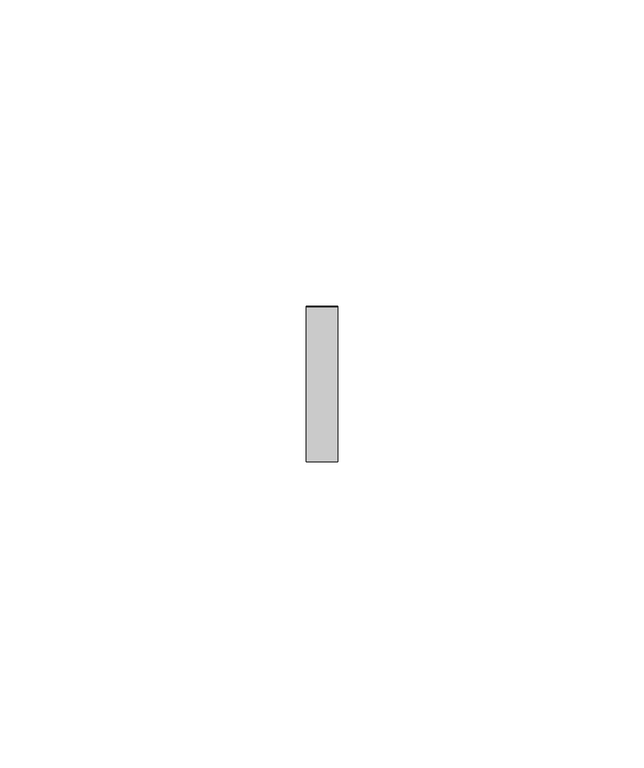
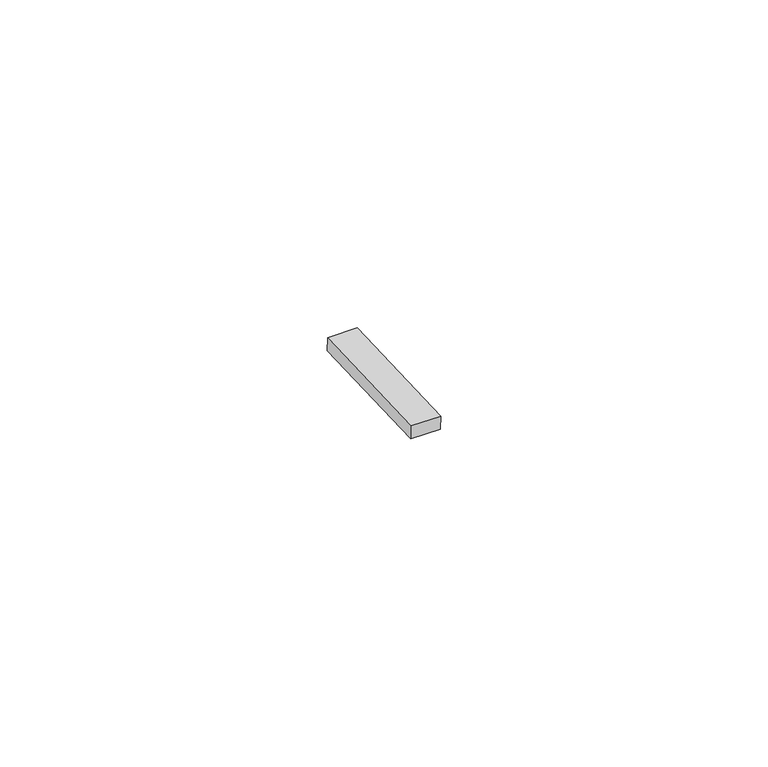
"""IFC4 building model written with IfcOpenShell, lengths in millimetres: proxy geometry, Inner panel:Inner panel:1:Inner panel:1 : Inner panel:Inner panel:300324:2:Inner panel:1:Inner panel:1 : Inner panel:Inner panel:300324:2 : Inner panel:Inner panel:1:Inner panel:1 : Inner panel:Inner panel:300324:300043:112 : Inner panel:Inner panel:1:Inner panel:1 : Inner panel:Inner panel:300324:2:Inner panel:1:Inner panel:1 : Inner panel:Inner panel:300324:2 : Inner panel:Inner panel:1:Inner panel:1 : Inner panel:Inner panel:300324:300043:308120."""

from ifc_helpers import new_model, si_unit, frame, origin, place, context, project, spatial, polyline, outline, extrude, source, transform, mapped, element, save


def generic_models_f19137aa(model_context):
    return source(origin(), model_context, "Body", "SweptSolid", [
        extrude(outline(polyline([(0.0, -25.3999999), (0.0, 0.0), (5.2138089, 0.0), (5.2138089, -25.3999999), (0.0, -25.3999999)])), frame((593936.595117, -578962.7476805, 3951.4793391), z_axis=(0.0, -0.041630544712223896, 0.9991330730923502), x_axis=(-1.0, 0.0, 0.0)), (0.0, 0.0, 1.0), 2.4763745),
    ])


if __name__ == "__main__":
    model = new_model("IFC4")
    model_context = context("Model", 3, world=origin())
    ifc_project = project(units=[si_unit("LENGTHUNIT", "METRE", prefix="MILLI")], contexts=[model_context])
    site = spatial("IfcSite", under=ifc_project)
    building = spatial("IfcBuilding", under=site)
    placement = place(None, origin())
    generic_models_shape = generic_models_f19137aa(model_context)
    element("IfcBuildingElementProxy", 1, Name="Inner panel:Inner panel:1:Inner panel:1 : Inner panel:Inner panel:300324:2:Inner panel:1:Inner panel:1 : Inner panel:Inner panel:300324:2 : Inner panel:Inner panel:1:Inner panel:1 : Inner panel:Inner panel:300324:300043:112 : Inner panel:Inner panel:1:Inner panel:1 : Inner panel:Inner panel:300324:2:Inner panel:1:Inner panel:1 : Inner panel:Inner panel:300324:2 : Inner panel:Inner panel:1:Inner panel:1 : Inner panel:Inner panel:300324:300043:308120", ObjectType="Inner panel:Inner panel:1:Inner panel:1 : Inner panel:Inner panel:300324:2:Inner panel:1:Inner panel:1 : Inner panel:Inner panel:300324:2 : Inner panel:Inner panel:1:Inner panel:1 : Inner panel:Inner panel:300324:300043:112 : Inner panel:Inner panel:1:Inner panel:1 : Inner panel:Inner panel:300324:2:Inner panel:1:Inner panel:1 : Inner panel:Inner panel:300324:2 : Inner panel:Inner panel:1:Inner panel:1 : Inner panel:Inner panel:300324:300043:308120", at=placement, inside=building, context=model_context, shape_type="MappedRepresentation", body=[
        mapped(generic_models_shape, transform((0.0, 0.0, 0.0), x_axis=(1.0, 0.0, 0.0), y_axis=(0.0, 1.0, 0.0), z_axis=(0.0, 0.0, 1.0))),
    ])
    save(model, "model.ifc")

# Revit data of these elements
# Type "Inner panel:Inner panel:1:Inner panel:1 : Inner panel:Inner panel:300324:2:Inner panel:1:Inner panel:1 : Inner panel:Inner panel:300324:2 : Inner panel:Inner panel:1:Inner panel:1 : Inner panel:Inner panel:300324:300043:112 : Inner panel:Inner panel:1:Inner panel:1 : Inner panel:Inner panel:300324:2:Inner panel:1:Inner panel:1 : Inner panel:Inner panel:300324:2 : Inner panel:Inner panel:1:Inner panel:1 : Inner panel:Inner panel:300324:300043:308120"
#   NameOverride = "Inner panel:Inner panel:1:Inner panel:1 : Inner panel:Inner panel:300324:2:Inner panel:1:Inner panel:1 : Inner panel:Inner panel:300324:2 : Inner panel:Inner panel:1:Inner panel:1 : Inner panel:Inner panel:300324:300043:308120"
#   ObjectTypeOverride = "Inner panel:1:Inner panel:1 : Inner panel:Inner panel:300324:2 : Inner panel:Inner panel:1:Inner panel:1 : Inner panel:Inner panel:300324:300043"
#   Reference = "Inner panel"
#   Tag = "308120"
# Element 1 (IfcBuildingElementProxy, "Inner panel:Inner panel:1:Inner panel:1 : Inner panel:Inner panel:300324:2:Inner panel:1:Inner panel:1 : Inner panel:Inner panel:300324:2 : Inner panel:Inner panel:1:Inner panel:1 : Inner panel:Inner panel:300324:300043:112 : Inner panel:Inner panel:1:Inner panel:1 : Inner panel:Inner panel:300324:2:Inner panel:1:Inner panel:1 : Inner panel:Inner panel:300324:2 : Inner panel:Inner panel:1:Inner panel:1 : Inner panel:Inner panel:300324:300043:308120")
#   Materials on its faces: "AT CLIP - 1\" WIDE NON ABSORBENT, WEATHER-RESISTANT NEOPRENE/EPDM/SBR FOAM"
# Materials
#   "AT CLIP - 1\" WIDE NON ABSORBENT, WEATHER-RESISTANT NEOPRENE/EPDM/SBR FOAM": class "Generic", colour RGB 85 85 85, transparency 0, Cost = 0
